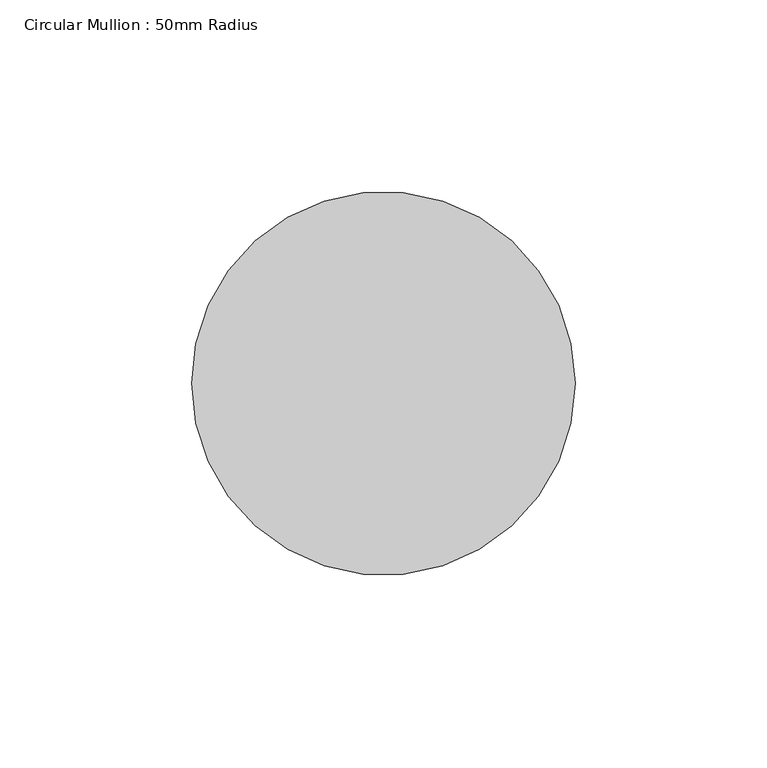
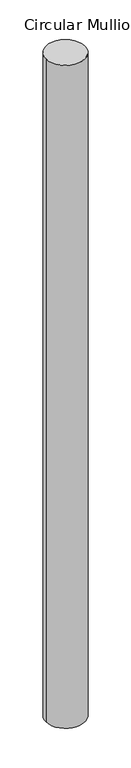
"""IFC4 building model written with IfcOpenShell, lengths in millimetres: member geometry, Circular Mullion : 50mm Radius."""

from ifc_helpers import new_model, si_unit, point, frame, origin, origin_2d, place, context, project, spatial, circle_curve, trimmed, segment, composite_curve, outline, extrude, source, transform, mapped, element, save


def circular_mullion_50mm_radius_b738f594(model_context):
    return source(origin(), model_context, "Body", "SweptSolid", [
        extrude(outline(composite_curve([segment(trimmed(circle_curve(origin_2d(), 50.0), [point((50.0, 0.0))], [point((-50.0, 0.0))], False, "CARTESIAN"), True, "CONTINUOUS"), segment(trimmed(circle_curve(origin_2d(), 50.0), [point((-50.0, 0.0))], [point((50.0, 0.0))], False, "CARTESIAN"), True, "CONTINUOUS")], self_intersect=False)), frame((0.0, 0.0, -1799.0942635), z_axis=(0.0, 0.0, 1.0), x_axis=(1.0, 0.0, 0.0)), (0.0, 0.0, 1.0), 1799.0942635),
    ])


if __name__ == "__main__":
    model = new_model("IFC4")
    model_context = context("Model", 3, world=origin())
    ifc_project = project(units=[si_unit("LENGTHUNIT", "METRE", prefix="MILLI")], contexts=[model_context])
    site = spatial("IfcSite", under=ifc_project)
    building = spatial("IfcBuilding", under=site)
    placement = place(None, origin())
    circular_mullion_50mm_radius_shape = circular_mullion_50mm_radius_b738f594(model_context)
    element("IfcMember", 1, ObjectType="Circular Mullion : 50mm Radius", at=placement, inside=building, context=model_context, shape_type="MappedRepresentation", body=[
        mapped(circular_mullion_50mm_radius_shape, transform((0.0, 0.0, 0.0), x_axis=(1.0, 0.0, 0.0), y_axis=(0.0, 1.0, 0.0), z_axis=(0.0, 0.0, 1.0))),
    ])
    save(model, "model.ifc")

# Revit data of these elements
# Type "Circular Mullion : 50mm Radius"
#   built-in parameter 1007350 = 0.164042 (stored number, unit not read)
# Element 1 (IfcMember, "Circular Mullion : 50mm Radius")
#   Materials on its faces: "Aluminium"
# Materials
#   "Aluminium": class "Metal", colour RGB 247 247 247, transparency 0, Description = "Aluminium 6061", Cost = 0
